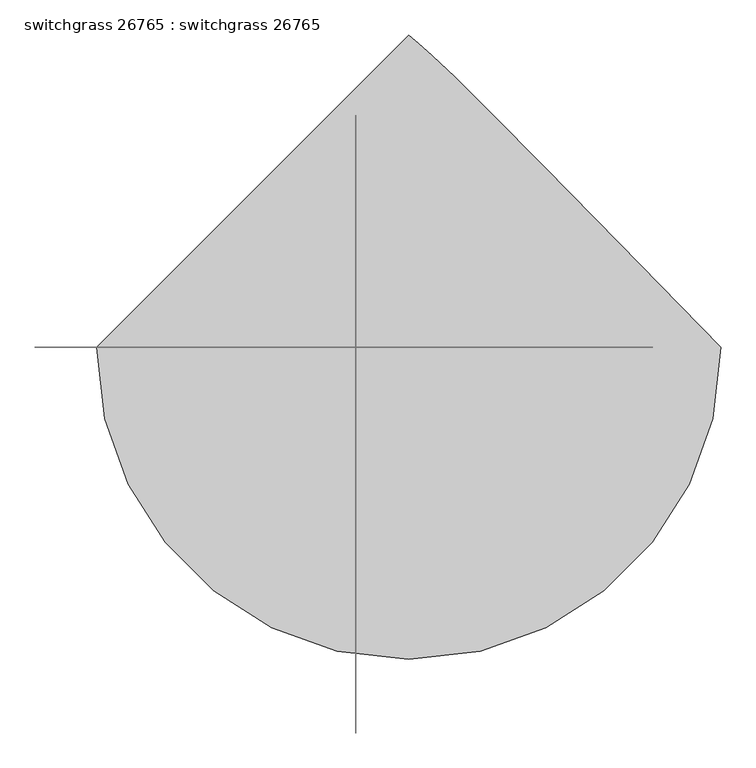
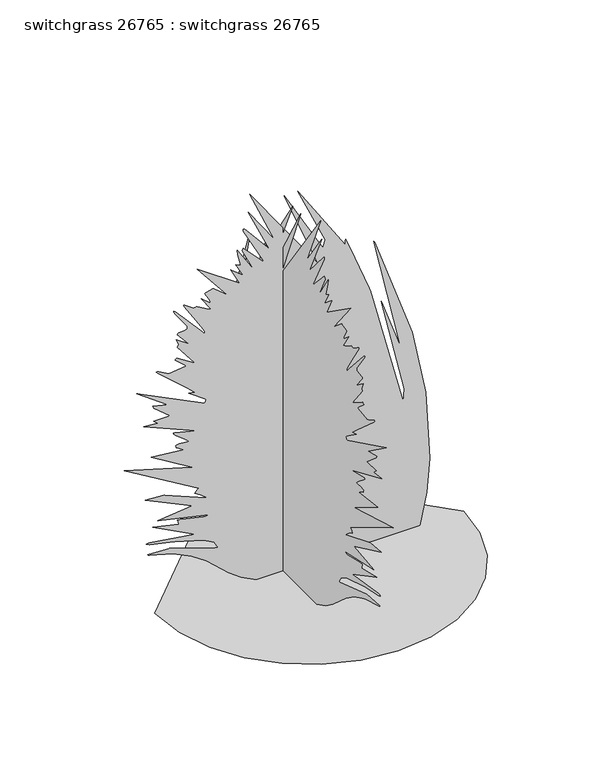
"""IFC4 building model written with IfcOpenShell, lengths in millimetres: proxy geometry, switchgrass 26765 : switchgrass 26765."""

from ifc_helpers import new_model, si_unit, origin, place, context, project, spatial, triangles, source, transform, mapped, element, save


def switchgrass_26765_switchgrass_26765_d4ad6bd8(model_context):
    return source(origin(), model_context, "Body", "Tessellation", [
        triangles([(-459.698612, 0.0, 4.65e-05), (-447.5447391, -105.3326149, 4.65e-05), (-412.9347513, -202.0637927, 4.65e-05), (-358.6347227, -287.4208646, 4.65e-05), (-287.4208646, -358.6372662, 4.65e-05), (-202.0637927, -412.9347513, 4.65e-05), (-105.3326149, -447.5447391, 4.65e-05), (2.01e-05, -459.698612, 4.65e-05), (105.3326149, -447.5447391, 4.65e-05), (202.0637927, -412.9347513, 4.65e-05), (287.4208646, -358.6347227, 4.65e-05), (358.6372662, -287.4208646, 4.65e-05), (412.9347513, -202.0637927, 4.65e-05), (447.5447391, -105.3326149, 4.65e-05), (459.698612, 4.02e-05, 4.65e-05), (310.3062409, 153.2394836, 4.65e-05), (199.5550432, 266.0620302, 4.65e-05), (121.0036242, 345.2057822, 4.65e-05), (68.212606, 397.4052123, 4.65e-05), (34.7415567, 429.3964645, 4.65e-05), (14.1507237, 447.915574, 4.65e-05), (-6.03e-05, 459.698612, 4.65e-05), (25.778164, 7.09e-05, 931.0228226), (-73.9743319, 5.62e-05, 1178.5581493), (40.5563681, 6.83e-05, 975.3584158), (47.9454701, 6.69e-05, 997.5250134), (-33.3343979, 5.62e-05, 1178.5581493), (107.0580365, 6.91e-05, 960.5807568), (108.009768, 6.88e-05, 974.8428223), (108.4339518, 6.88e-05, 976.8163937), (108.9381361, 6.87e-05, 977.5631504), (121.537794, 7.04e-05, 948.2515675), (179.4161744, 7.78e-05, 798.7728281), (181.6249422, 7.82e-05, 791.64056), (280.7025792, 0.0001022, 406.3993581), (283.3568685, 9.98e-05, 447.039283), (214.1996435, 8.19e-05, 746.2965254), (273.311188, 9.18e-05, 580.0436282), (192.0325918, 7.02e-05, 942.1073204), (195.7270065, 7.05e-05, 938.4116884), (306.5800512, 8.97e-05, 615.8245474), (346.866909, 0.0001017, 413.7119931), (359.1935185, 0.0001144, 200.6111561), (350.2374882, 0.0001206, 97.2772745), (328.7313518, 0.0001264, 3.02e-05), (-155.9468584, 0.0001256, 0.034436), (-202.0081638, 0.0001242, 22.9207712), (-238.8497922, 0.0001227, 50.4692123), (-306.8086347, 0.0001194, 111.5848133), (-348.8913131, 0.0001178, 141.1673826), (-403.686624, 0.0001164, 167.4436493), (-477.2830038, 0.0001152, 188.5593844), (-477.9662833, 0.0001151, 188.9317636), (-478.6673306, 0.0001151, 189.4758256), (-479.3200888, 0.0001151, 190.1286019), (-479.8636602, 0.000115, 190.8281231), (-480.2344952, 0.000115, 191.5116207), (-480.3742032, 0.000115, 192.1161441), (-413.8720124, 0.0001152, 188.421475), (-269.7856765, 0.000118, 140.3924299), (-282.1148113, 0.0001168, 160.9176305), (-313.8012674, 0.0001157, 178.5812689), (-403.4097877, 0.0001139, 205.4826247), (-474.9589087, 0.000113, 221.4147554), (-484.0673281, 0.000113, 225.3669851), (-481.6365535, 0.000113, 227.0964581), (-478.1059914, 0.0001131, 227.7690551), (-473.780347, 0.0001131, 227.6730399), (-339.9809921, 0.0001141, 206.8940938), (-465.5965078, 0.0001101, 273.3949947), (-388.0097829, 0.0001112, 254.9241563), (-391.5657795, 0.0001104, 268.675697), (-391.7054875, 0.0001103, 269.7018517), (-378.6955985, 0.0001105, 267.1821653), (-313.5091704, 0.0001114, 252.3912622), (-310.4256014, 0.0001114, 251.228706), (-299.3410672, 0.0001112, 254.9241563), (-450.816269, 0.0001092, 288.1752335), (-347.369858, 0.0001086, 299.2572424), (-487.7630327, 0.0001046, 365.7593968), (-432.3454124, 0.0001048, 362.0637285), (-306.7298967, 0.0001079, 310.3417766), (-306.6994117, 0.0001078, 311.3857172), (-309.3435817, 0.0001077, 314.1746458), (-314.0120831, 0.0001074, 318.1928962), (-320.0598244, 0.0001072, 322.9223677), (-333.6919501, 0.0001066, 332.4448242), (-339.9809921, 0.0001064, 336.2040061), (-339.5619043, 0.0001063, 337.0523918), (-332.7115231, 0.0001059, 344.2304057), (-328.896458, 0.0001057, 347.2860332), (-550.5695189, 9.78e-05, 480.2903784), (-347.369858, 0.0001013, 421.1770535), (-469.2896327, 9.69e-05, 495.0680737), (-373.2320875, 9.76e-05, 483.9835396), (-374.0728065, 9.75e-05, 484.9741405), (-391.8451592, 9.68e-05, 496.840967), (-395.3986124, 9.67e-05, 498.7637784), (-395.5967471, 9.66e-05, 499.9347098), (-396.9810376, 9.65e-05, 504.0037565), (-397.0470946, 9.64e-05, 505.1086673), (-396.5848045, 9.63e-05, 505.8681413), (-395.3986124, 9.62e-05, 506.1526079), (-391.824848, 9.63e-05, 507.3895964), (-386.3283085, 9.63e-05, 507.7426635), (-361.3779056, 9.63e-05, 505.9697339), (-358.4543921, 9.62e-05, 506.1526079), (-365.3428525, 9.57e-05, 513.0766402), (-398.2154826, 9.31e-05, 538.6416859), (-403.0567205, 9.28e-05, 543.2873689), (-404.6620005, 9.27e-05, 546.7493669), (-400.0315782, 9.31e-05, 546.74428), (-336.2878309, 9.47e-05, 532.0148375), (-491.4561939, 9.07e-05, 598.5144848), (-450.816269, 9.09e-05, 594.8213236), (-458.7029606, 9.05e-05, 601.7732975), (-461.4817154, 9.03e-05, 605.0168859), (-461.9008032, 9.03e-05, 605.9033143), (-413.8720124, 9.03e-05, 605.9033143), (-461.9008032, 8.79e-05, 646.5432392), (-465.5965078, 8.74e-05, 653.9346485), (-421.2608783, 8.81e-05, 642.850078), (-513.6252623, 8.41e-05, 709.3522688), (-310.4256014, 9.01e-05, 609.599019), (-306.7298967, 8.94e-05, 620.6835531), (-358.4543921, 8.72e-05, 657.6278097), (-339.9809921, 8.74e-05, 653.9346485), (-364.4437068, 8.67e-05, 676.0859854), (-450.3971449, 8.26e-05, 751.897201), (-454.5119373, 8.13e-05, 757.3810959), (-451.4106005, 8.15e-05, 757.7264963), (-446.9833998, 8.18e-05, 756.2457001), (-417.5677171, 8.24e-05, 738.9076595), (-367.3392786, 8.19e-05, 745.9485815), (-365.8432217, 8.19e-05, 746.2965254), (-399.0943171, 8.02e-05, 775.8519161), (-398.8123939, 8.01e-05, 776.4208494), (-398.0529199, 8.01e-05, 777.091448), (-396.9480091, 8e-05, 777.7924953), (-394.2302244, 8e-05, 779.0167665), (-392.876419, 7.99e-05, 779.4028622), (-391.7054875, 7.99e-05, 779.5476208), (-342.833398, 8.18e-05, 747.6173023), (-339.9809921, 8.19e-05, 746.2965254), (-391.7054875, 7.8e-05, 812.7987162), (-388.0097829, 7.75e-05, 820.187582), (-395.3986124, 7.64e-05, 838.6609457), (-358.4543921, 7.8e-05, 812.7987162), (-391.7054875, 7.55e-05, 853.4386047), (-391.1365179, 7.55e-05, 854.4724079), (-390.4684991, 7.54e-05, 855.4528713), (-389.7649083, 7.54e-05, 856.3113945), (-389.0994329, 7.53e-05, 856.9742901), (-388.5406371, 7.53e-05, 857.3807333), (-388.1545415, 7.53e-05, 857.454348), (-388.0097829, 7.53e-05, 857.1343094), (-371.4439336, 7.53e-05, 857.9572969), (-366.4147347, 7.52e-05, 859.1713943), (-363.3692811, 7.51e-05, 861.0890825), (-362.1704081, 7.49e-05, 863.8297583), (-362.6758641, 7.47e-05, 867.5178326), (-364.7484847, 7.44e-05, 872.2777891), (-398.1672297, 7.28e-05, 919.6461914), (-402.3683905, 7.2e-05, 927.1721855), (-402.7874783, 7.09e-05, 931.0228226), (-397.8573286, 7.11e-05, 927.2000908), (-324.6191028, 7.61e-05, 844.1930208), (-310.4256014, 7.71e-05, 827.5763752), (-310.4256014, 7.78e-05, 835.1430645), (-320.710039, 7.69e-05, 852.757905), (-345.0991027, 7.52e-05, 891.1626829), (-371.9874687, 7.2e-05, 934.0708197), (-373.2320875, 7.05e-05, 938.4116884), (-370.2628284, 7.08e-05, 937.8046034), (-365.6527173, 7.1e-05, 935.328083), (-343.6766968, 7.16e-05, 919.9407955), (-341.8986803, 7.15e-05, 920.3700571), (-337.7610332, 7.15e-05, 920.8247532), (-335.7900052, 7.15e-05, 920.8373978), (-334.1441028, 7.15e-05, 920.6977261), (-333.0112504, 7.15e-05, 920.4005785), (-332.5921626, 7.16e-05, 919.9407955), (-299.1302334, 7.27e-05, 900.3193188), (-294.3855376, 7.29e-05, 898.213706), (-291.9522195, 7.29e-05, 897.7717272), (-321.5075921, 7.02e-05, 942.1073204), (-295.647906, 7.16e-05, 919.9407955), (-294.9392465, 7.14e-05, 922.478286), (-296.4556329, 7.11e-05, 927.3702839), (-299.4274173, 7.08e-05, 933.6441015), (-310.4256014, 6.96e-05, 953.1918909), (-307.5325367, 6.95e-05, 954.7641787), (-286.1407102, 6.92e-05, 960.3648542), (-284.5633718, 6.91e-05, 960.5807568), (-243.9231744, 7.11e-05, 927.3296614), (-332.5921626, 6.45e-05, 1038.1649019), (-206.9776643, 6.98e-05, 949.4961863), (-232.8394033, 6.67e-05, 1001.2206453), (-231.0110992, 6.68e-05, 1000.0979668), (-195.8941475, 6.85e-05, 971.6627111), (-218.0614536, 6.61e-05, 1012.3026724), (-203.2832495, 6.65e-05, 1004.9138065), (-212.5006375, 6.44e-05, 1040.9334829), (-214.4800588, 6.35e-05, 1054.5479136), (-214.3667663, 6.34e-05, 1056.6383383), (-162.6433064, 6.83e-05, 975.3584158), (-199.5885623, 6.39e-05, 1049.2494724), (-195.8941475, 6.34e-05, 1056.6383383), (-136.7815765, 6.72e-05, 993.8318521), (-136.7815765, 6.77e-05, 997.1490915), (-195.320854, 6.02e-05, 1109.0105049), (-195.8941475, 5.99e-05, 1115.7516632), (-191.8857621, 6.01e-05, 1114.2327152), (-118.3086943, 6.52e-05, 1027.0829475), (-181.1159253, 5.7e-05, 1163.7804176), (-103.5307446, 6.36e-05, 1052.9426336), (-177.4215105, 5.37e-05, 1219.1980379), (-77.7843237, 7.9038071, 931.0228226), (-77.7843237, -91.8487905, 1178.5581493), (-77.7843237, 22.6819595, 975.3584158), (-77.7843237, 30.0710115, 997.5250134), (-77.7843237, -51.2088565, 1178.5581493), (-77.7843237, 89.1835734, 960.5807568), (-77.7843237, 90.1355684, 974.8428223), (-77.7843237, 90.5594887, 976.8163937), (-77.7843237, 91.0636821, 977.5631504), (-77.7843237, 103.6633309, 948.2515675), (-77.7843237, 161.5417022, 798.7728281), (-77.7843237, 163.7507425, 791.64056), (-77.7843237, 262.8260722, 406.3993581), (-77.7843237, 265.4829231, 447.039283), (-77.7843237, 196.3254257, 746.2965254), (-77.7843237, 255.4372245, 580.0436282), (-77.7843237, 174.1581196, 942.1073204), (-77.7843237, 177.8525525, 938.4116884), (-77.7843237, 288.7035625, 615.8245474), (-77.7843237, 328.9929637, 413.7119931), (-77.7843237, 341.3195732, 200.6111561), (-77.7843237, 332.3635428, 97.2772745), (-77.7843237, 310.854863, 0.0), (-77.7843237, -173.8213124, 0.0344058), (-77.7843237, -219.8826179, 22.9207462), (-77.7843237, -256.7250093, 50.4692123), (-77.7843237, -324.6826163, 111.5848133), (-77.7843237, -366.7652584, 141.1673826), (-77.7843237, -421.5605693, 167.4436493), (-77.7843237, -495.1569855, 188.5593844), (-77.7843237, -495.8402287, 188.9317636), (-77.7843237, -496.541276, 189.4758256), (-77.7843237, -497.1940341, 190.1286019), (-77.7843237, -497.7376056, 190.8281231), (-77.7843237, -498.1109839, 191.5113845), (-77.7843237, -498.2481485, 192.1161441), (-77.7843237, -431.7459578, 188.421475), (-77.7843237, -287.6596218, 140.3924299), (-77.7843237, -299.9887566, 160.9176305), (-77.7843237, -331.6752128, 178.5812689), (-77.7843237, -421.283733, 205.4826247), (-77.7843237, -492.8328541, 221.4147554), (-77.7843237, -501.9438532, 225.3669851), (-77.7843237, -499.5105351, 227.0964581), (-77.7843237, -495.9824801, 227.7690551), (-77.7843237, -491.6543286, 227.6730399), (-77.7843237, -357.8549375, 206.8940938), (-77.7843237, -483.4704532, 273.3949947), (-77.7843237, -405.8837282, 254.9241563), (-77.7843237, -409.4422683, 268.675697), (-77.7843237, -409.5794329, 269.7018517), (-77.7843237, -396.5695802, 267.1821653), (-77.7843237, -331.3831158, 252.3912622), (-77.7843237, -328.2995467, 251.228706), (-77.7843237, -317.2150126, 254.9241563), (-77.7843237, -468.6927578, 288.1752335), (-77.7843237, -365.2438033, 299.2572424), (-77.7843237, -505.6369781, 365.7593968), (-77.7843237, -450.2193578, 362.0637285), (-77.7843237, -324.6038784, 310.3417766), (-77.7843237, -324.5733933, 311.3857172), (-77.7843237, -327.217527, 314.1746458), (-77.7843237, -331.8885718, 318.1928962), (-77.7843237, -337.9337697, 322.9223677), (-77.7843237, -351.5659318, 332.4448242), (-77.7843237, -357.8549375, 336.2040061), (-77.7843237, -357.4358497, 337.0523918), (-77.7843237, -350.5854684, 344.2304057), (-77.7843237, -346.7729467, 347.2860332), (-77.7843237, -568.4434642, 480.2903784), (-77.7843237, -365.2438033, 421.1770535), (-77.7843237, -487.1636144, 495.0680737), (-77.7843237, -391.1060328, 483.9835396), (-77.7843237, -391.9467882, 484.9741405), (-77.7843237, -409.7191409, 496.840967), (-77.7843237, -413.2725941, 498.7637784), (-77.7843237, -413.4706924, 499.9347098), (-77.7843237, -414.8549829, 504.0037565), (-77.7843237, -414.92104, 505.1086673), (-77.7843237, -414.4587499, 505.8681413), (-77.7843237, -413.2725941, 506.1526079), (-77.7843237, -409.6987933, 507.3895964), (-77.7843237, -404.2022538, 507.7426635), (-77.7843237, -379.2518872, 505.9697339), (-77.7843237, -376.3283375, 506.1526079), (-77.7843237, -383.2167978, 513.0766402), (-77.7843237, -416.0894279, 538.6416859), (-77.7843237, -420.9306659, 543.2873689), (-77.7843237, -422.5359458, 546.7493669), (-77.7843237, -417.9055235, 546.74428), (-77.7843237, -354.1617763, 532.0148375), (-77.7843237, -509.3326827, 598.5144848), (-77.7843237, -468.6927578, 594.8213236), (-77.7843237, -476.5769059, 601.7732975), (-77.7843237, -479.3556607, 605.0168859), (-77.7843237, -479.7747485, 605.9033143), (-77.7843237, -431.7459578, 605.9033143), (-77.7843237, -479.7747485, 646.5432392), (-77.7843237, -483.4704532, 653.9346485), (-77.7843237, -439.1348236, 642.850078), (-77.7843237, -531.4992439, 709.3522688), (-77.7843237, -328.2995467, 609.599019), (-77.7843237, -324.6038784, 620.6835531), (-77.7843237, -376.3283375, 657.6278097), (-77.7843237, -357.8549375, 653.9346485), (-77.7843237, -382.3176521, 676.0859854), (-77.7843237, -468.2711266, 751.897201), (-77.7843237, -472.385919, 757.3810959), (-77.7843237, -469.2845821, 757.7264963), (-77.7843237, -464.8573451, 756.2457001), (-77.7843237, -435.4416624, 738.9076595), (-77.7843237, -385.2132603, 745.9485815), (-77.7843237, -383.7172033, 746.2965254), (-77.7843237, -416.9682624, 775.8544596), (-77.7843237, -416.6863392, 776.4208494), (-77.7843237, -415.9268652, 777.091448), (-77.7843237, -414.8245342, 777.7924953), (-77.7843237, -412.1041698, 779.0167665), (-77.7843237, -410.7529078, 779.4028622), (-77.7843237, -409.5794329, 779.5476208), (-77.7843237, -360.7098867, 747.6173023), (-77.7843237, -357.8549375, 746.2965254), (-77.7843237, -409.5794329, 812.7987162), (-77.7843237, -405.8837282, 820.187582), (-77.7843237, -413.2725941, 838.6609457), (-77.7843237, -376.3283375, 812.7987162), (-77.7843237, -409.5794329, 853.4386047), (-77.7843237, -409.0104632, 854.4724079), (-77.7843237, -408.3424444, 855.4528713), (-77.7843237, -407.6413971, 856.3113945), (-77.7843237, -406.9759217, 856.9742901), (-77.7843237, -406.4145824, 857.3807333), (-77.7843237, -406.0285232, 857.454348), (-77.7843237, -405.8837282, 857.1343094), (-77.7843237, -389.3204224, 857.9572969), (-77.7843237, -384.2912235, 859.1713943), (-77.7843237, -381.2432264, 861.0890825), (-77.7843237, -380.0443534, 863.8297583), (-77.7843237, -380.5498095, 867.5178326), (-77.7843237, -382.62243, 872.2803326), (-77.7843237, -416.0411751, 919.6461914), (-77.7843237, -420.2423358, 927.1721855), (-77.7843237, -420.663967, 931.0228226), (-77.7843237, -415.7313103, 927.2000908), (-77.7843237, -342.4955915, 844.1930208), (-77.7843237, -328.2995467, 827.5763752), (-77.7843237, -328.2995467, 835.1430645), (-77.7843237, -338.5839844, 852.757905), (-77.7843237, -362.973048, 891.1626829), (-77.7843237, -389.8639938, 934.0708197), (-77.7843237, -391.1060328, 938.4116884), (-77.7843237, -388.1367737, 937.8046034), (-77.7843237, -383.526699, 935.328083), (-77.7843237, -361.5506421, 919.9407955), (-77.7843237, -359.772662, 920.3700571), (-77.7843237, -355.6375219, 920.8247532), (-77.7843237, -353.666494, 920.8373978), (-77.7843237, -352.0180481, 920.6977261), (-77.7843237, -350.8877392, 920.4005785), (-77.7843237, -350.4661079, 919.9407955), (-77.7843237, -317.0041969, 900.3193188), (-77.7843237, -312.2594647, 898.213706), (-77.7843237, -309.8261467, 897.7717272), (-77.7843237, -339.3815738, 942.1073204), (-77.7843237, -313.5218513, 919.9407955), (-77.7843237, -312.81321, 922.478286), (-77.7843237, -314.3295782, 927.3702839), (-77.7843237, -317.3013808, 933.6441015), (-77.7843237, -328.2995467, 953.1918909), (-77.7843237, -325.406482, 954.7641787), (-77.7843237, -304.0146555, 960.3648542), (-77.7843237, -302.4373172, 960.5807568), (-77.7843237, -261.7973741, 927.3296614), (-77.7843237, -350.4661079, 1038.1649019), (-77.7843237, -224.8521183, 949.4961863), (-77.7843237, -250.7138573, 1001.2206453), (-77.7843237, -248.8855714, 1000.0979668), (-77.7843237, -213.7686015, 971.6627111), (-77.7843237, -235.9356533, 1012.3026724), (-77.7843237, -221.1577035, 1004.9138065), (-77.7843237, -230.3750915, 1040.9334829), (-77.7843237, -232.3545128, 1054.5479136), (-77.7843237, -232.2412203, 1056.6383383), (-77.7843237, -180.5177605, 975.3584158), (-77.7843237, -217.4630163, 1049.2494724), (-77.7843237, -213.7686015, 1056.6383383), (-77.7843237, -154.6557853, 993.8318521), (-77.7843237, -154.6557853, 997.1490915), (-77.7843237, -213.1953262, 1109.0105049), (-77.7843237, -213.7686015, 1115.7516632), (-77.7843237, -209.7602343, 1114.2327152), (-77.7843237, -136.1831483, 1027.0829475), (-77.7843237, -198.9903975, 1163.7804176), (-77.7843237, -121.4049442, 1052.9426336), (-77.7843237, -195.2957102, 1219.1980379)], [[21, 22, 1], [20, 21, 1], [19, 20, 1], [18, 19, 1], [17, 18, 1], [17, 1, 2], [17, 2, 3], [17, 3, 4], [16, 17, 4], [16, 4, 5], [16, 5, 6], [16, 6, 7], [16, 7, 8], [16, 8, 9], [16, 9, 10], [16, 10, 11], [16, 11, 12], [15, 16, 12], [14, 15, 12], [13, 14, 12], [36, 37, 38], [23, 24, 25], [26, 27, 28], [122, 123, 124], [214, 215, 216], [216, 217, 23], [69, 70, 71], [91, 92, 93], [185, 186, 187], [195, 196, 197], [113, 114, 115], [77, 78, 79], [79, 80, 81], [79, 81, 82], [125, 126, 127], [93, 94, 95], [197, 198, 199], [38, 39, 40], [38, 40, 41], [146, 147, 148], [200, 201, 202], [204, 205, 206], [203, 204, 206], [202, 203, 206], [200, 202, 206], [164, 165, 166], [120, 121, 122], [119, 120, 122], [36, 38, 41], [36, 41, 42], [30, 31, 32], [29, 30, 32], [28, 29, 32], [77, 79, 82], [64, 65, 66], [64, 66, 67], [129, 130, 131], [197, 199, 200], [163, 164, 166], [129, 131, 132], [119, 122, 124], [64, 67, 68], [172, 173, 174], [211, 212, 213], [117, 118, 119], [116, 117, 119], [115, 116, 119], [113, 115, 119], [113, 119, 124], [110, 111, 112], [35, 36, 42], [207, 208, 209], [206, 207, 209], [72, 73, 74], [57, 58, 59], [56, 57, 59], [55, 56, 59], [54, 55, 59], [53, 54, 59], [52, 53, 59], [51, 52, 59], [51, 59, 60], [50, 51, 60], [49, 50, 60], [214, 216, 23], [25, 26, 28], [162, 163, 166], [162, 166, 167], [161, 162, 167], [160, 161, 167], [211, 213, 214], [210, 211, 214], [48, 49, 60], [172, 174, 175], [171, 172, 175], [190, 191, 192], [63, 64, 68], [63, 68, 69], [62, 63, 69], [109, 110, 112], [87, 88, 89], [129, 132, 133], [210, 214, 23], [209, 210, 23], [23, 25, 28], [108, 109, 112], [108, 112, 113], [107, 108, 113], [171, 175, 176], [44, 45, 46], [145, 146, 148], [144, 145, 148], [154, 155, 156], [135, 136, 137], [135, 137, 138], [135, 138, 139], [135, 139, 140], [135, 140, 141], [135, 141, 142], [135, 142, 143], [43, 44, 46], [171, 176, 177], [171, 177, 178], [171, 178, 179], [171, 179, 180], [171, 180, 181], [171, 181, 182], [171, 182, 183], [170, 171, 183], [170, 183, 184], [170, 184, 185], [42, 43, 46], [35, 42, 46], [35, 46, 47], [35, 47, 48], [35, 48, 60], [35, 60, 61], [34, 35, 61], [34, 61, 62], [34, 62, 69], [148, 149, 150], [148, 150, 151], [148, 151, 152], [148, 152, 153], [148, 153, 154], [148, 154, 156], [148, 156, 157], [148, 157, 158], [159, 160, 167], [148, 158, 159], [148, 159, 167], [148, 167, 168], [144, 148, 168], [128, 129, 133], [128, 133, 134], [128, 134, 135], [128, 135, 143], [128, 143, 144], [169, 170, 185], [71, 72, 74], [69, 71, 74], [69, 74, 75], [69, 75, 76], [23, 28, 32], [33, 34, 69], [197, 200, 206], [206, 209, 23], [190, 192, 193], [190, 193, 194], [190, 194, 195], [189, 190, 195], [188, 189, 195], [187, 188, 195], [185, 187, 195], [87, 89, 90], [87, 90, 91], [97, 98, 99], [127, 128, 144], [86, 87, 91], [23, 32, 33], [101, 102, 103], [100, 101, 103], [100, 103, 104], [99, 100, 104], [97, 99, 104], [97, 104, 105], [96, 97, 105], [96, 105, 106], [95, 96, 106], [95, 106, 107], [93, 95, 107], [93, 107, 113], [125, 127, 144], [197, 206, 23], [169, 185, 195], [69, 76, 77], [33, 69, 77], [33, 77, 82], [33, 82, 83], [33, 83, 84], [33, 84, 85], [33, 85, 86], [33, 86, 91], [33, 91, 93], [33, 93, 113], [33, 113, 124], [33, 124, 125], [33, 125, 144], [33, 144, 168], [23, 33, 168], [197, 23, 168], [195, 197, 168], [169, 195, 168], [231, 232, 233], [218, 219, 220], [221, 222, 223], [317, 318, 319], [409, 410, 411], [411, 412, 218], [264, 265, 266], [286, 287, 288], [380, 381, 382], [390, 391, 392], [308, 309, 310], [272, 273, 274], [274, 275, 276], [274, 276, 277], [320, 321, 322], [288, 289, 290], [392, 393, 394], [233, 234, 235], [233, 235, 236], [341, 342, 343], [395, 396, 397], [399, 400, 401], [398, 399, 401], [397, 398, 401], [395, 397, 401], [359, 360, 361], [315, 316, 317], [314, 315, 317], [231, 233, 236], [231, 236, 237], [225, 226, 227], [224, 225, 227], [223, 224, 227], [272, 274, 277], [259, 260, 261], [259, 261, 262], [324, 325, 326], [392, 394, 395], [358, 359, 361], [324, 326, 327], [314, 317, 319], [259, 262, 263], [367, 368, 369], [406, 407, 408], [312, 313, 314], [311, 312, 314], [310, 311, 314], [308, 310, 314], [308, 314, 319], [305, 306, 307], [230, 231, 237], [402, 403, 404], [401, 402, 404], [267, 268, 269], [252, 253, 254], [251, 252, 254], [250, 251, 254], [249, 250, 254], [248, 249, 254], [247, 248, 254], [246, 247, 254], [246, 254, 255], [245, 246, 255], [244, 245, 255], [409, 411, 218], [220, 221, 223], [357, 358, 361], [357, 361, 362], [356, 357, 362], [355, 356, 362], [406, 408, 409], [405, 406, 409], [243, 244, 255], [367, 369, 370], [366, 367, 370], [385, 386, 387], [258, 259, 263], [258, 263, 264], [257, 258, 264], [304, 305, 307], [282, 283, 284], [324, 327, 328], [405, 409, 218], [404, 405, 218], [218, 220, 223], [303, 304, 307], [303, 307, 308], [302, 303, 308], [366, 370, 371], [239, 240, 241], [340, 341, 343], [339, 340, 343], [349, 350, 351], [330, 331, 332], [330, 332, 333], [330, 333, 334], [330, 334, 335], [330, 335, 336], [330, 336, 337], [330, 337, 338], [238, 239, 241], [366, 371, 372], [366, 372, 373], [366, 373, 374], [366, 374, 375], [366, 375, 376], [366, 376, 377], [366, 377, 378], [365, 366, 378], [365, 378, 379], [365, 379, 380], [237, 238, 241], [230, 237, 241], [230, 241, 242], [230, 242, 243], [230, 243, 255], [230, 255, 256], [229, 230, 256], [229, 256, 257], [229, 257, 264], [343, 344, 345], [343, 345, 346], [343, 346, 347], [343, 347, 348], [343, 348, 349], [343, 349, 351], [343, 351, 352], [343, 352, 353], [354, 355, 362], [343, 353, 354], [343, 354, 362], [343, 362, 363], [339, 343, 363], [323, 324, 328], [323, 328, 329], [323, 329, 330], [323, 330, 338], [323, 338, 339], [364, 365, 380], [266, 267, 269], [264, 266, 269], [264, 269, 270], [264, 270, 271], [218, 223, 227], [228, 229, 264], [392, 395, 401], [401, 404, 218], [385, 387, 388], [385, 388, 389], [385, 389, 390], [384, 385, 390], [383, 384, 390], [382, 383, 390], [380, 382, 390], [282, 284, 285], [282, 285, 286], [292, 293, 294], [322, 323, 339], [281, 282, 286], [218, 227, 228], [296, 297, 298], [295, 296, 298], [295, 298, 299], [294, 295, 299], [292, 294, 299], [292, 299, 300], [291, 292, 300], [291, 300, 301], [290, 291, 301], [290, 301, 302], [288, 290, 302], [288, 302, 308], [320, 322, 339], [392, 401, 218], [364, 380, 390], [264, 271, 272], [228, 264, 272], [228, 272, 277], [228, 277, 278], [228, 278, 279], [228, 279, 280], [228, 280, 281], [228, 281, 286], [228, 286, 288], [228, 288, 308], [228, 308, 319], [228, 319, 320], [228, 320, 339], [228, 339, 363], [218, 228, 363], [392, 218, 363], [390, 392, 363], [364, 390, 363]], closed=False),
    ])


if __name__ == "__main__":
    model = new_model("IFC4")
    model_context = context("Model", 3, world=origin())
    ifc_project = project(units=[si_unit("LENGTHUNIT", "METRE", prefix="MILLI")], contexts=[model_context])
    site = spatial("IfcSite", under=ifc_project)
    building = spatial("IfcBuilding", under=site)
    placement = place(None, origin())
    switchgrass_26765_switchgrass_26765_shape = switchgrass_26765_switchgrass_26765_d4ad6bd8(model_context)
    element("IfcBuildingElementProxy", 1, Name="switchgrass 26765 : switchgrass 26765", ObjectType="switchgrass 26765 : switchgrass 26765", at=placement, inside=building, context=model_context, shape_type="MappedRepresentation", body=[
        mapped(switchgrass_26765_switchgrass_26765_shape, transform((0.0, 0.0, 0.0), x_axis=(1.0, 0.0, 0.0), y_axis=(0.0, 1.0, 0.0), z_axis=(0.0, 0.0, 1.0))),
    ])
    save(model, "model.ifc")

# Revit data of these elements
# Type "switchgrass 26765 : switchgrass 26765"
#   built-in parameter 1005195 = "RPC-16-FVP6-6SQ0-2RXK-S000-ST1L-LVER-AU"
#   Height = 0
